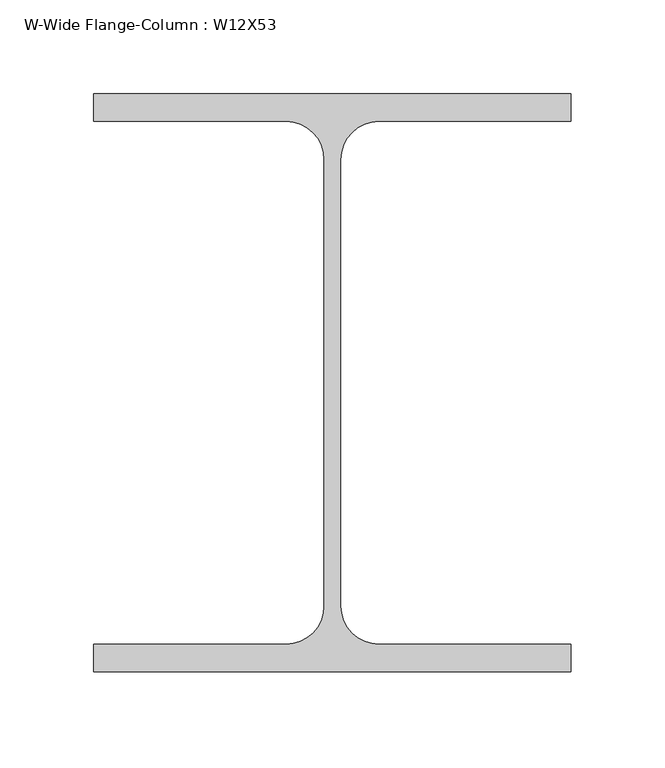
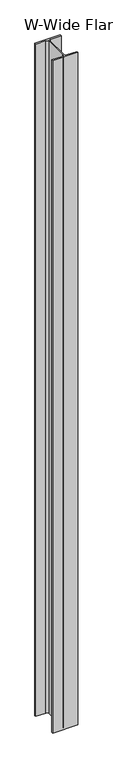
"""IFC4 building model written with IfcOpenShell, lengths in millimetres: column geometry, W-Wide Flange-Column : W12X53."""

import ifcopenshell
import ifcopenshell.guid

model = None  # the IFC model being written
_history = None  # IfcOwnerHistory: only IFC2X3 demands one
_inside = {}  # id of a spatial element -> (the spatial element, [elements in it])
_under = {}  # id of a project, library or spatial element -> (it, [spatial elements below it])
_declared = {}  # id of a project -> (the project, [libraries it declares])
_typed = {}  # id of a type object -> (the type object, [elements of that type])
_made_of = {}  # id of a material, layer set ... -> (it, [elements and type objects made of it])


def new_model(schema):
    """Start an empty IFC model of exactly this schema.

    Asked for "IFC4X3", IfcOpenShell would pick the latest addendum, in which some entities
    have other attributes; the version numbers below select the first issue.
    IFC2X3 requires an IfcOwnerHistory on every rooted entity: one is made here for all.
    """
    global model, _history
    if schema == "IFC4X3":
        model = ifcopenshell.file(schema_version=(4, 3, 0, 0))
    else:
        model = ifcopenshell.file(schema=schema)
    _inside.clear()
    _under.clear()
    _declared.clear()
    _typed.clear()
    _made_of.clear()
    _history = None
    if model.schema == "IFC2X3":
        org = make("IfcOrganization", Name="unknown")
        user = make(
            "IfcPersonAndOrganization",
            ThePerson=make("IfcPerson", FamilyName="unknown"),
            TheOrganization=org,
        )
        app = make(
            "IfcApplication",
            ApplicationDeveloper=org,
            Version="unknown",
            ApplicationFullName="unknown",
            ApplicationIdentifier="unknown",
        )
        _history = make(
            "IfcOwnerHistory",
            OwningUser=user,
            OwningApplication=app,
            ChangeAction="ADDED",
            CreationDate=0,
        )
    return model


def make(cls, **values):
    """One entity of the class cls with the attributes given. An attribute that is None is left unset."""
    return model.create_entity(
        cls, **{name: value for name, value in values.items() if value is not None}
    )


def rooted(cls, **values):
    """An entity with a GlobalId (a new one), such as an element, a storey or a relation."""
    return make(cls, GlobalId=ifcopenshell.guid.new(), OwnerHistory=_history, **values)


def si_unit(unit_type, name, prefix=None):
    """IfcSIUnit, for example si_unit("LENGTHUNIT", "METRE", prefix="MILLI")."""
    return make("IfcSIUnit", UnitType=unit_type, Prefix=prefix, Name=name)


def assignment(units):
    """IfcUnitAssignment: the units of a project."""
    return None if units is None else make("IfcUnitAssignment", Units=units)


def point(xyz):
    """IfcCartesianPoint."""
    return None if xyz is None else make("IfcCartesianPoint", Coordinates=xyz)


def direction(xyz):
    """IfcDirection."""
    return None if xyz is None else make("IfcDirection", DirectionRatios=xyz)


def frame(location, z_axis=None, x_axis=None):
    """IfcAxis2Placement3D, a coordinate frame: its origin and axes. An axis left out is left unset."""
    return make(
        "IfcAxis2Placement3D",
        Location=point(location),
        Axis=direction(z_axis),
        RefDirection=direction(x_axis),
    )


def frame_2d(location, x_axis=None):
    """IfcAxis2Placement2D, a coordinate frame in the plane: its origin and x axis."""
    return make(
        "IfcAxis2Placement2D", Location=point(location), RefDirection=direction(x_axis)
    )


def origin():
    """The frame at (0, 0, 0) with its axes left unset."""
    return frame((0.0, 0.0, 0.0))


def place(relative_to, where):
    """IfcLocalPlacement: puts the frame where relative to a parent placement (None: the world)."""
    return make(
        "IfcLocalPlacement", PlacementRelTo=relative_to, RelativePlacement=where
    )


def context(
    kind, dimensions, precision=None, world=None, true_north=None, identifier=None
):
    """IfcGeometricRepresentationContext, for example the 3D "Model" context."""
    return make(
        "IfcGeometricRepresentationContext",
        ContextIdentifier=identifier,
        ContextType=kind,
        CoordinateSpaceDimension=dimensions,
        Precision=precision,
        WorldCoordinateSystem=world,
        TrueNorth=true_north,
    )


def project(units=None, contexts=None):
    """IfcProject with its units and contexts."""
    return rooted(
        "IfcProject",
        Name="project",
        RepresentationContexts=contexts,
        UnitsInContext=assignment(units),
    )


def spatial(cls, under=None, at=None, **own):
    """A site, building, storey or space (cls), placed at a placement, below another one or the project."""
    s = rooted(cls, ObjectPlacement=at, **own)
    if under is not None:
        _under.setdefault(under.id(), (under, []))[1].append(s)
    return s


def polyline(points):
    """IfcPolyline through the points."""
    return make("IfcPolyline", Points=[point(p) for p in points])


def circle_curve(where, radius):
    """IfcCircle in the frame where."""
    return make("IfcCircle", Position=where, Radius=radius)


def trimmed(basis, trim1, trim2, sense, master):
    """IfcTrimmedCurve: the piece of a basis curve between two trims."""
    return make(
        "IfcTrimmedCurve",
        BasisCurve=basis,
        Trim1=trim1,
        Trim2=trim2,
        SenseAgreement=sense,
        MasterRepresentation=master,
    )


def segment(curve, same_sense, transition):
    """IfcCompositeCurveSegment."""
    return make(
        "IfcCompositeCurveSegment",
        Transition=transition,
        SameSense=same_sense,
        ParentCurve=curve,
    )


def composite_curve(segments, self_intersect=None):
    """IfcCompositeCurve: segments joined end to end."""
    return make("IfcCompositeCurve", Segments=segments, SelfIntersect=self_intersect)


def outline(outer, holes=None, kind="AREA"):
    """IfcArbitraryClosedProfileDef: a profile drawn as a closed curve; with holes, ...WithVoids."""
    if holes is None:
        return make("IfcArbitraryClosedProfileDef", ProfileType=kind, OuterCurve=outer)
    return make(
        "IfcArbitraryProfileDefWithVoids",
        ProfileType=kind,
        OuterCurve=outer,
        InnerCurves=holes,
    )


def extrude(swept, where, along, depth):
    """IfcExtrudedAreaSolid: the profile swept, set in the frame where, extruded along a direction by depth."""
    return make(
        "IfcExtrudedAreaSolid",
        SweptArea=swept,
        Position=where,
        ExtrudedDirection=direction(along),
        Depth=depth,
    )


def shape(context_of_items, identifier, shape_type, items):
    """IfcShapeRepresentation: the items that make up one representation, for example the "Body"."""
    return make(
        "IfcShapeRepresentation",
        ContextOfItems=context_of_items,
        RepresentationIdentifier=identifier,
        RepresentationType=shape_type,
        Items=items,
    )


def source(mapping_origin, context_of_items, identifier, shape_type, items):
    """IfcRepresentationMap: a shape defined once, which mapped items show again and again."""
    return make(
        "IfcRepresentationMap",
        MappingOrigin=mapping_origin,
        MappedRepresentation=shape(context_of_items, identifier, shape_type, items),
    )


def transform(
    local_origin,
    x_axis=None,
    y_axis=None,
    z_axis=None,
    scale=None,
    scale2=None,
    scale3=None,
    uniform=True,
):
    """IfcCartesianTransformationOperator3D, or its non-uniform kind. x_axis, y_axis, z_axis: its Axis1, 2, 3."""
    if uniform:
        return make(
            "IfcCartesianTransformationOperator3D",
            Axis1=direction(x_axis),
            Axis2=direction(y_axis),
            LocalOrigin=point(local_origin),
            Scale=scale,
            Axis3=direction(z_axis),
        )
    return make(
        "IfcCartesianTransformationOperator3DnonUniform",
        Axis1=direction(x_axis),
        Axis2=direction(y_axis),
        LocalOrigin=point(local_origin),
        Scale=scale,
        Axis3=direction(z_axis),
        Scale2=scale2,
        Scale3=scale3,
    )


def mapped(mapping_source, mapping_target):
    """IfcMappedItem: shows the shape of a source again, moved by a transform."""
    return make(
        "IfcMappedItem", MappingSource=mapping_source, MappingTarget=mapping_target
    )


def made_of(thing, what):
    """Note that an element or type object is made of a material, layer set ...; save() writes the relation."""
    if what is not None:
        _made_of.setdefault(what.id(), (what, []))[1].append(thing)
    return thing


def element(
    cls,
    number,
    at=None,
    inside=None,
    cuts=None,
    type_object=None,
    material=None,
    context=None,
    identifier="Body",
    shape_type=None,
    held_by="IfcProductDefinitionShape",
    body=None,
    shapes=None,
    **own,
):
    """One element of the class cls, such as IfcWall. Its Tag is "e" and its number.

    at: its placement. inside: the storey or other place that contains it. cuts: it is an
    opening in that element (IfcRelVoidsElement). A single representation is given by context,
    identifier, shape_type and body (its items); several are given by shapes. held_by: the class
    of the entity that holds the representations. save() writes the other relations.
    """
    e = rooted(cls, Tag="e%d" % number, ObjectPlacement=at, **own)
    if body is not None:
        shapes = [shape(context, identifier, shape_type, body)]
    if shapes is not None:
        e.Representation = make(held_by, Representations=shapes)
    if inside is not None:
        _inside.setdefault(inside.id(), (inside, []))[1].append(e)
    if cuts is not None:
        rooted(
            "IfcRelVoidsElement", RelatingBuildingElement=cuts, RelatedOpeningElement=e
        )
    if type_object is not None:
        _typed.setdefault(type_object.id(), (type_object, []))[1].append(e)
    return made_of(e, material)


def aggregate(whole, parts):
    """IfcRelAggregates: a whole, such as a stair, and the parts it consists of."""
    return rooted("IfcRelAggregates", RelatingObject=whole, RelatedObjects=parts)


def save(model, path):
    """Write the relations noted so far, then the file.

    IfcRelAggregates (storeys below a building ...), IfcRelContainedInSpatialStructure (elements
    in a storey), IfcRelDefinesByType, IfcRelAssociatesMaterial and IfcRelDeclares: one each for
    every whole, place, type object, material and project.
    """
    for whole, parts in _under.values():
        aggregate(whole, parts)
    for where, things in _inside.values():
        rooted(
            "IfcRelContainedInSpatialStructure",
            RelatedElements=things,
            RelatingStructure=where,
        )
    for kind, things in _typed.values():
        rooted("IfcRelDefinesByType", RelatedObjects=things, RelatingType=kind)
    for what, things in _made_of.values():
        rooted("IfcRelAssociatesMaterial", RelatedObjects=things, RelatingMaterial=what)
    for by, libraries in _declared.values():
        rooted("IfcRelDeclares", RelatingContext=by, RelatedDefinitions=libraries)
    model.write(path)


def w_wide_flange_column_w12x53_9f3dc712(model_context):
    return source(origin(), model_context, "Body", "SweptSolid", [
        extrude(outline(composite_curve([segment(polyline([(127.0, 153.67), (127.0, 139.065), (24.7015, 139.065)]), True, "CONTINUOUS"), segment(trimmed(circle_curve(frame_2d((24.7015, 118.745)), 20.32), [point((24.7015, 139.065))], [point((4.3815, 118.745))], True, "CARTESIAN"), True, "CONTINUOUS"), segment(polyline([(4.3815, 118.745), (4.3815, -118.745)]), True, "CONTINUOUS"), segment(trimmed(circle_curve(frame_2d((24.7015, -118.745)), 20.32), [point((4.3815, -118.745))], [point((24.7015, -139.065))], True, "CARTESIAN"), True, "CONTINUOUS"), segment(polyline([(24.7015, -139.065), (127.0, -139.065), (127.0, -153.67), (-127.0, -153.67), (-127.0, -139.065), (-24.7015, -139.065)]), True, "CONTINUOUS"), segment(trimmed(circle_curve(frame_2d((-24.7015, -118.745)), 20.32), [point((-24.7015, -139.065))], [point((-4.3815, -118.745))], True, "CARTESIAN"), True, "CONTINUOUS"), segment(polyline([(-4.3815, -118.745), (-4.3815, 118.745)]), True, "CONTINUOUS"), segment(trimmed(circle_curve(frame_2d((-24.7015, 118.745)), 20.32), [point((-4.3815, 118.745))], [point((-24.7015, 139.065))], True, "CARTESIAN"), True, "CONTINUOUS"), segment(polyline([(-24.7015, 139.065), (-127.0, 139.065), (-127.0, 153.67), (127.0, 153.67)]), True, "CONTINUOUS")], self_intersect=False)), frame((0.0, 0.0, 8756.65), z_axis=(0.0, 0.0, 1.0), x_axis=(1.0, 0.0, 0.0)), (0.0, 0.0, 1.0), 7146.3296875),
    ])


if __name__ == "__main__":
    model = new_model("IFC4")
    model_context = context("Model", 3, world=origin())
    ifc_project = project(units=[si_unit("LENGTHUNIT", "METRE", prefix="MILLI")], contexts=[model_context])
    site = spatial("IfcSite", under=ifc_project)
    building = spatial("IfcBuilding", under=site)
    placement = place(None, origin())
    w_wide_flange_column_w12x53_shape = w_wide_flange_column_w12x53_9f3dc712(model_context)
    element("IfcColumn", 1, ObjectType="W-Wide Flange-Column : W12X53", at=placement, inside=building, context=model_context, shape_type="MappedRepresentation", body=[
        mapped(w_wide_flange_column_w12x53_shape, transform((0.0, 0.0, 0.0), x_axis=(1.0, 0.0, 0.0), y_axis=(0.0, 1.0, 0.0), z_axis=(0.0, 0.0, 1.0))),
    ])
    save(model, "model.ifc")

# Revit data of these elements
# Type "W-Wide Flange-Column : W12X53"
#   Assembly Code = "B10"
#   W = 53
#   bf = 0' - 10"
#   d = 1' - 0.1"
#   k = 0' - 1 3/8"
#   kr = 0' - 0.8"
#   tf = 0' - 0.575"
#   tw = 0' - 0.345"
#   A = 0.108333 SF
#   Structural Material [instance default] = Steel ASTM A992
# Element 1 (IfcColumn, "W-Wide Flange-Column : W12X53")
#   Materials on its faces: "Steel ASTM A992"
# Materials
#   "Steel ASTM A992": class "Metal", colour RGB 199 199 199, transparency 0, Description = "Structural steel 50ksi", Cost = 0
